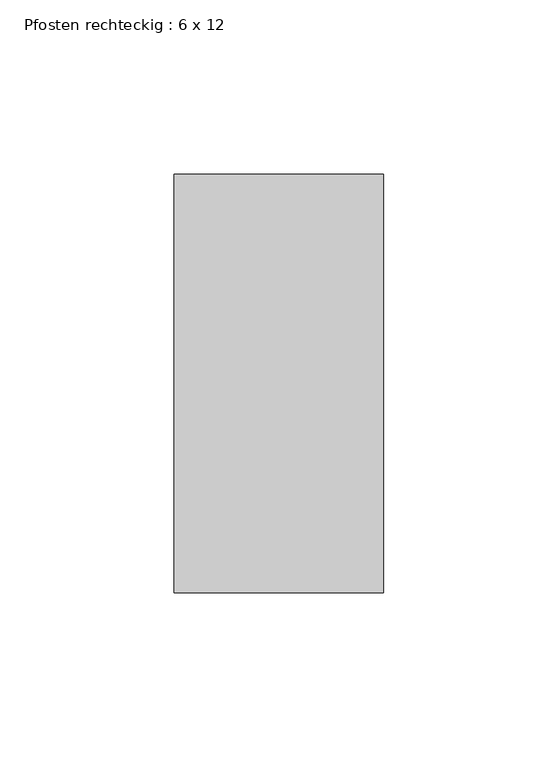
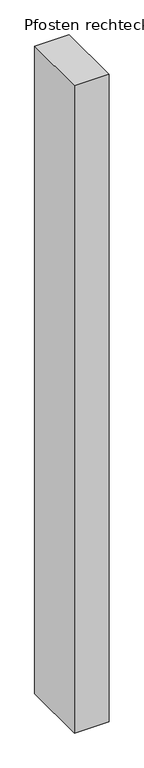
"""IFC4 building model written with IfcOpenShell, lengths in millimetres: member geometry, Pfosten rechteckig : 6 x 12."""

from ifc_helpers import new_model, si_unit, frame, origin, place, context, project, spatial, polyline, outline, extrude, source, transform, mapped, element, save


def pfosten_rechteckig_6_x_12_36a2a28f(model_context):
    return source(origin(), model_context, "Body", "SweptSolid", [
        extrude(outline(polyline([(0.0, 60.0), (0.0, -60.0), (-60.0, -60.0), (-60.0, 60.0), (0.0, 60.0)])), frame((0.0, 0.0, -1190.0), z_axis=(0.0, 0.0, 1.0), x_axis=(1.0, 0.0, 0.0)), (0.0, 0.0, 1.0), 1190.0),
    ])


if __name__ == "__main__":
    model = new_model("IFC4")
    model_context = context("Model", 3, world=origin())
    ifc_project = project(units=[si_unit("LENGTHUNIT", "METRE", prefix="MILLI")], contexts=[model_context])
    site = spatial("IfcSite", under=ifc_project)
    building = spatial("IfcBuilding", under=site)
    placement = place(None, origin())
    pfosten_rechteckig_6_x_12_shape = pfosten_rechteckig_6_x_12_36a2a28f(model_context)
    element("IfcMember", 1, ObjectType="Pfosten rechteckig : 6 x 12", at=placement, inside=building, context=model_context, shape_type="MappedRepresentation", body=[
        mapped(pfosten_rechteckig_6_x_12_shape, transform((0.0, 0.0, 0.0), x_axis=(1.0, 0.0, 0.0), y_axis=(0.0, 1.0, 0.0), z_axis=(0.0, 0.0, 1.0))),
    ])
    save(model, "model.ifc")

# Revit data of these elements
# Type "Pfosten rechteckig : 6 x 12"
#   built-in parameter 1007304 = 0.393701 (stored number, unit not read)
#   built-in parameter 1007301 = 0.0984252 (stored number, unit not read)
#   built-in parameter 1007300 = 0.0984252 (stored number, unit not read)
# Element 1 (IfcMember, "Pfosten rechteckig : 6 x 12")
#   Materials on its faces: "Metall - verzinkt"
# Materials
#   "Metall - verzinkt": class "Allgemeines", colour RGB 200 200 200, transparency 0, Cost = 0
